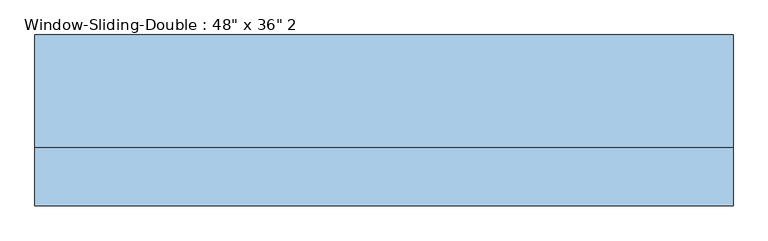
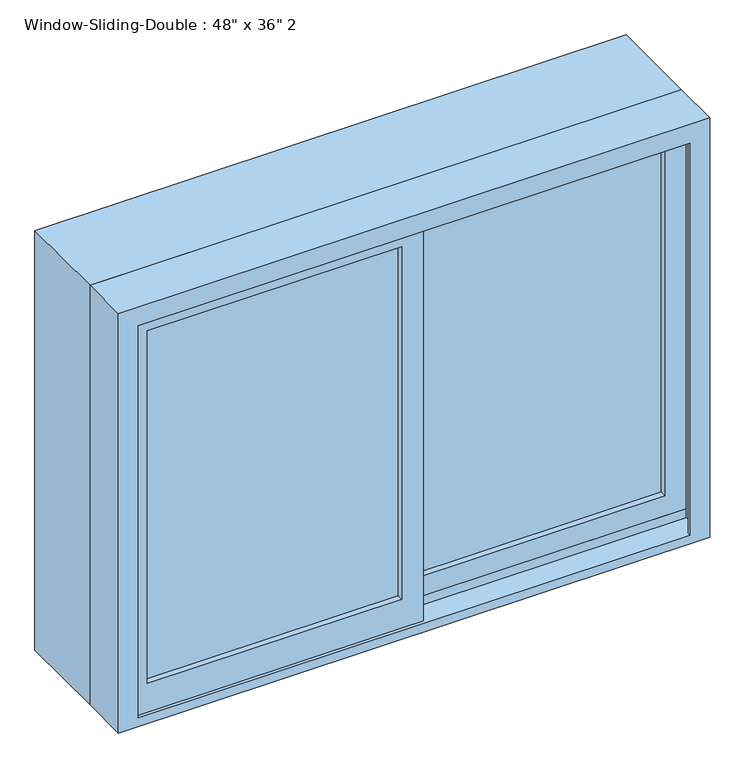
"""IFC4 building model written with IfcOpenShell, lengths in millimetres: window geometry."""

from ifc_helpers import new_model, si_unit, frame, origin, place, context, project, spatial, polyline, outline, extrude, faceted_brep, source, transform, mapped, element, save


def window_32be7210(model_context):
    return source(origin(), model_context, "Body", "SolidModel", [
        faceted_brep([(-609.6, -53.34, 914.4), (609.6, -53.34, 914.4), (609.6, -154.94, 914.4), (-609.6, -154.94, 914.4), (-568.6778905, -154.94, 1787.8778905), (-568.6778905, -154.94, 933.45), (-568.6778905, -148.59, 933.45), (-568.6778905, -148.59, 1787.8778905), (-590.55, -148.59, 933.45), (-590.55, -148.59, 1809.75), (590.55, -148.59, 1809.75), (590.55, -148.59, 933.45), (568.6778905, -148.59, 933.45), (568.6778905, -148.59, 1787.8778905), (-590.55, -104.14, 933.45), (-590.55, -104.14, 952.5), (-590.55, -59.69, 952.5), (-590.55, -59.69, 933.45), (-590.55, -53.34, 933.45), (-590.55, -53.34, 1809.75), (-609.6, -53.34, 1828.8), (609.6, -53.34, 1828.8), (590.55, -53.34, 1809.75), (590.55, -53.34, 933.45), (-609.6, -154.94, 1828.8), (609.6, -154.94, 1828.8), (568.6778905, -154.94, 1787.8778905), (568.6778905, -154.94, 933.45), (590.55, -59.69, 933.45), (590.55, -59.69, 952.5), (590.55, -104.14, 952.5), (590.55, -104.14, 933.45)], [[[0, 1, 2, 3]], [[4, 5, 6, 7]], [[7, 6, 8, 9, 10, 11, 12, 13]], [[9, 8, 14, 15, 16, 17, 18, 19]], [[0, 20, 21, 1], [22, 19, 18, 23]], [[24, 20, 0, 3]], [[2, 25, 24, 3], [4, 26, 27, 5]], [[7, 13, 26, 4]], [[9, 19, 22, 10]], [[20, 24, 25, 21]], [[13, 12, 27, 26]], [[22, 23, 28, 29, 30, 31, 11, 10]], [[21, 25, 2, 1]], [[27, 12, 11, 31, 14, 8, 6, 5]], [[31, 30, 15, 14]], [[30, 29, 16, 15]], [[29, 28, 17, 16]], [[18, 17, 28, 23]]]),
        extrude(outline(polyline([(1828.8, 609.6), (1828.8, -609.6), (914.4, -609.6), (914.4, 609.6), (1828.8, 609.6)]), holes=[polyline([(1809.75, -590.55), (1809.75, 590.55), (933.45, 590.55), (933.45, -590.55), (1809.75, -590.55)])]), frame((0.0, -53.34, 0.0), z_axis=(0.0, 1.0, 0.0), x_axis=(0.0, 0.0, 1.0)), (0.0, 0.0, 1.0), 196.85),
        extrude(outline(polyline([(546.1, -91.44), (22.225, -91.44), (22.225, -85.09), (546.1, -85.09), (546.1, -91.44)])), frame((0.0, 0.0, 996.95), z_axis=(0.0, 0.0, 1.0), x_axis=(1.0, 0.0, 0.0)), (0.0, 0.0, 1.0), 768.35),
        extrude(outline(polyline([(546.1, -78.74), (22.225, -78.74), (22.225, -72.39), (546.1, -72.39), (546.1, -78.74)])), frame((0.0, 0.0, 996.95), z_axis=(0.0, 0.0, 1.0), x_axis=(1.0, 0.0, 0.0)), (0.0, 0.0, 1.0), 768.35),
        extrude(outline(polyline([(-22.225, -135.89), (-546.1, -135.89), (-546.1, -129.54), (-22.225, -129.54), (-22.225, -135.89)])), frame((0.0, 0.0, 996.95), z_axis=(0.0, 0.0, 1.0), x_axis=(1.0, 0.0, 0.0)), (0.0, 0.0, 1.0), 768.35),
        extrude(outline(polyline([(-22.225, -123.19), (-546.1, -123.19), (-546.1, -116.84), (-22.225, -116.84), (-22.225, -123.19)])), frame((0.0, 0.0, 996.95), z_axis=(0.0, 0.0, 1.0), x_axis=(1.0, 0.0, 0.0)), (0.0, 0.0, 1.0), 768.35),
        extrude(outline(polyline([(933.45, 22.225), (1809.75, 22.225), (1809.75, -590.55), (933.45, -590.55), (933.45, 22.225)]), holes=[polyline([(1765.3, -546.1), (1765.3, -22.225), (996.95, -22.225), (996.95, -546.1), (1765.3, -546.1)])]), frame((0.0, -148.59, 0.0), z_axis=(0.0, 1.0, 0.0), x_axis=(0.0, 0.0, 1.0)), (0.0, 0.0, 1.0), 44.45),
        extrude(outline(polyline([(952.5, -22.225), (952.5, 590.55), (1809.75, 590.55), (1809.75, -22.225), (952.5, -22.225)]), holes=[polyline([(996.95, 546.1), (996.95, 22.225), (1765.3, 22.225), (1765.3, 546.1), (996.95, 546.1)])]), frame((0.0, -104.14, 0.0), z_axis=(0.0, 1.0, 0.0), x_axis=(0.0, 0.0, 1.0)), (0.0, 0.0, 1.0), 44.45),
    ])


if __name__ == "__main__":
    model = new_model("IFC4")
    model_context = context("Model", 3, world=origin())
    ifc_project = project(units=[si_unit("LENGTHUNIT", "METRE", prefix="MILLI")], contexts=[model_context])
    site = spatial("IfcSite", under=ifc_project)
    building = spatial("IfcBuilding", under=site)
    placement = place(None, origin())
    window_shape = window_32be7210(model_context)
    element("IfcWindow", 1, ObjectType="Window-Sliding-Double : 48\" x 36\" 2", at=placement, inside=building, context=model_context, shape_type="MappedRepresentation", body=[
        mapped(window_shape, transform((0.0, 0.0, 0.0), x_axis=(1.0, 0.0, 0.0), y_axis=(0.0, 1.0, 0.0), z_axis=(0.0, 0.0, 1.0))),
    ])
    save(model, "model.ifc")

# Revit data of these elements
# Type "Window-Sliding-Double : 48\" x 36\" 2"
#   Type Mark = "16"
#   Fire Rating = "0.5h"
#   Assembly Code = "B2020100"
#   Analytic Construction = "Double glazing - domestic"
#   Window Inset [instance default] = 0' - 0"
#   Wall Thickness [instance default] = 0' - 6"
#   Visual Light Transmittance = 0.81
#   Thermal Resistance (R) = 0.319569 (m²·K)/W
#   Solar Heat Gain Coefficient = 0.76
#   Muntin Width = 1' - 8 5/8"
#   Muntin Height = 2' - 6 1/4"
#   Interior Wall Closure [instance default] = 0' - 2 3/4"
#   Heat Transfer Coefficient (U) = 3.12929 W/(m²·K)
#   Frame Extension [instance default] = 0' - 0 1/4"
#   Exterior Wall Closure [instance default] = 0' - 1 1/4"
#   Rough Width = 4' - 0 1/2"
#   Rough Height = 3' - 0 1/2"
#   Height = 3' - 0"
#   Extension Jamb [instance default] = 0' - 2 3/4"
#   Default Sill Height = 3' - 0"
#   Width = 4' - 0"
#   Interior Trim Visibility [instance default] = yes
#   Indicator Visibility [instance default] = yes
#   Exterior Trim Visibility [instance default] = yes
#   Muntin Visibility = no
#   Extension Jamb Visibility [instance default] = yes
#   Muntin Pattern = Muntin Pattern_2x2 : Muntin Pattern_2x2
#   Interior Trim Material = Wood - Stained
#   Interior Trim = Trim-Window-Interior-Flat : Picture Frame
#   Interior Frame Material = Wood - Stained
#   Glass Panel Material = Glass
#   Exterior Trim Material = Clad - White
#   Exterior Trim = Trim-Window-Exterior-Flat : with Sill
#   Exterior Frame Material = Clad - White
#   Wall Closure = (empty or 0)
# Element 1 (IfcWindow, "Window-Sliding-Double : 48\" x 36\" 2")
#   Wall Thickness = 0' - 11"
#   Extension Jamb = 0' - 7 3/4"
#   Materials on its faces: "Wood - Stained", "Glass", "Clad - White"
# Materials
#   "Wood - Stained": class "Wood", colour RGB 224 178 126, transparency 0, Cost = 0
#   "Glass": class "Glass", colour RGB 218 227 224, transparency 0.57, Description = "Soda Lime Glass", Cost = 0
#   "Clad - White": class "Wood", colour RGB 242 242 238, transparency 0, Cost = 0
